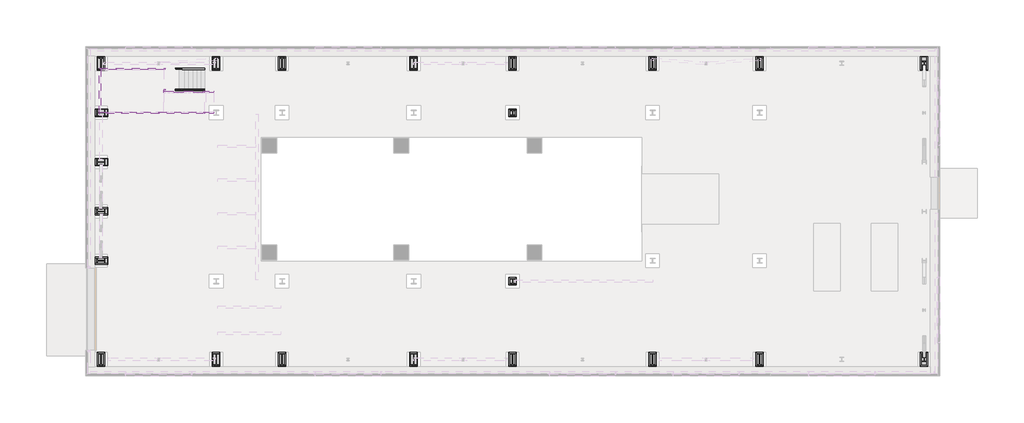
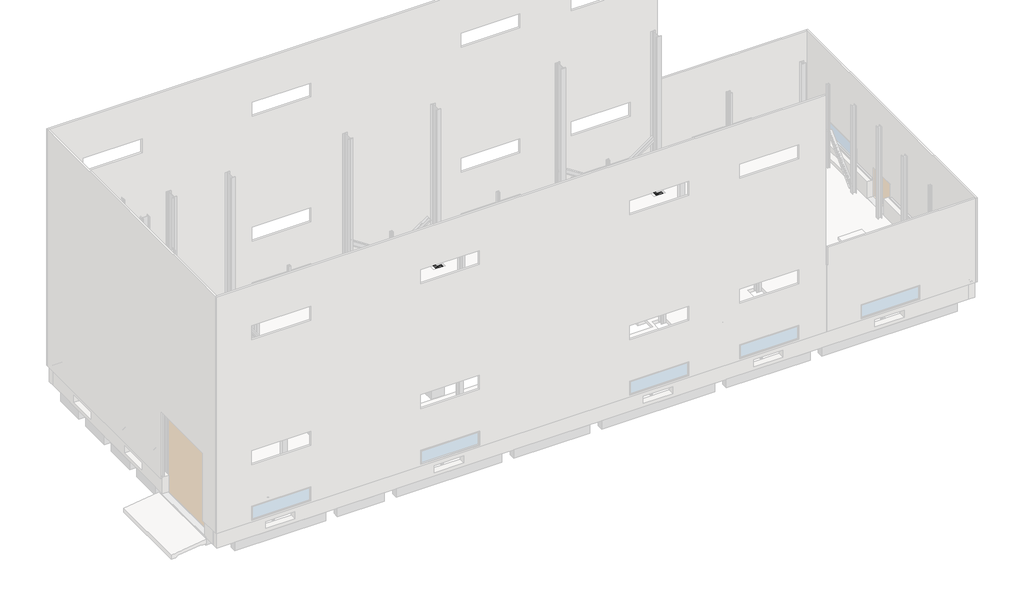
# One storey, part 4 of 4: 23 proxies, 10 members.
"""IFC4 building model written with IfcOpenShell, lengths in millimetres."""

import ifcopenshell
import ifcopenshell.guid

model = None  # the IFC model being written
_history = None  # IfcOwnerHistory: only IFC2X3 demands one
_inside = {}  # id of a spatial element -> (the spatial element, [elements in it])
_under = {}  # id of a project, library or spatial element -> (it, [spatial elements below it])
_declared = {}  # id of a project -> (the project, [libraries it declares])
_typed = {}  # id of a type object -> (the type object, [elements of that type])
_made_of = {}  # id of a material, layer set ... -> (it, [elements and type objects made of it])


def new_model(schema):
    """Start an empty IFC model of exactly this schema.

    Asked for "IFC4X3", IfcOpenShell would pick the latest addendum, in which some entities
    have other attributes; the version numbers below select the first issue.
    IFC2X3 requires an IfcOwnerHistory on every rooted entity: one is made here for all.
    """
    global model, _history
    if schema == "IFC4X3":
        model = ifcopenshell.file(schema_version=(4, 3, 0, 0))
    else:
        model = ifcopenshell.file(schema=schema)
    _inside.clear()
    _under.clear()
    _declared.clear()
    _typed.clear()
    _made_of.clear()
    _history = None
    if model.schema == "IFC2X3":
        org = make("IfcOrganization", Name="unknown")
        user = make(
            "IfcPersonAndOrganization",
            ThePerson=make("IfcPerson", FamilyName="unknown"),
            TheOrganization=org,
        )
        app = make(
            "IfcApplication",
            ApplicationDeveloper=org,
            Version="unknown",
            ApplicationFullName="unknown",
            ApplicationIdentifier="unknown",
        )
        _history = make(
            "IfcOwnerHistory",
            OwningUser=user,
            OwningApplication=app,
            ChangeAction="ADDED",
            CreationDate=0,
        )
    return model


def make(cls, **values):
    """One entity of the class cls with the attributes given. An attribute that is None is left unset."""
    return model.create_entity(
        cls, **{name: value for name, value in values.items() if value is not None}
    )


def rooted(cls, **values):
    """An entity with a GlobalId (a new one), such as an element, a storey or a relation."""
    return make(cls, GlobalId=ifcopenshell.guid.new(), OwnerHistory=_history, **values)


def si_unit(unit_type, name, prefix=None):
    """IfcSIUnit, for example si_unit("LENGTHUNIT", "METRE", prefix="MILLI")."""
    return make("IfcSIUnit", UnitType=unit_type, Prefix=prefix, Name=name)


def assignment(units):
    """IfcUnitAssignment: the units of a project."""
    return None if units is None else make("IfcUnitAssignment", Units=units)


def point(xyz):
    """IfcCartesianPoint."""
    return None if xyz is None else make("IfcCartesianPoint", Coordinates=xyz)


def direction(xyz):
    """IfcDirection."""
    return None if xyz is None else make("IfcDirection", DirectionRatios=xyz)


def frame(location, z_axis=None, x_axis=None):
    """IfcAxis2Placement3D, a coordinate frame: its origin and axes. An axis left out is left unset."""
    return make(
        "IfcAxis2Placement3D",
        Location=point(location),
        Axis=direction(z_axis),
        RefDirection=direction(x_axis),
    )


def frame_2d(location, x_axis=None):
    """IfcAxis2Placement2D, a coordinate frame in the plane: its origin and x axis."""
    return make(
        "IfcAxis2Placement2D", Location=point(location), RefDirection=direction(x_axis)
    )


def origin():
    """The frame at (0, 0, 0) with its axes left unset."""
    return frame((0.0, 0.0, 0.0))


def place(relative_to, where):
    """IfcLocalPlacement: puts the frame where relative to a parent placement (None: the world)."""
    return make(
        "IfcLocalPlacement", PlacementRelTo=relative_to, RelativePlacement=where
    )


def context(
    kind, dimensions, precision=None, world=None, true_north=None, identifier=None
):
    """IfcGeometricRepresentationContext, for example the 3D "Model" context."""
    return make(
        "IfcGeometricRepresentationContext",
        ContextIdentifier=identifier,
        ContextType=kind,
        CoordinateSpaceDimension=dimensions,
        Precision=precision,
        WorldCoordinateSystem=world,
        TrueNorth=true_north,
    )


def project(units=None, contexts=None):
    """IfcProject with its units and contexts."""
    return rooted(
        "IfcProject",
        Name="project",
        RepresentationContexts=contexts,
        UnitsInContext=assignment(units),
    )


def spatial(cls, under=None, at=None, **own):
    """A site, building, storey or space (cls), placed at a placement, below another one or the project."""
    s = rooted(cls, ObjectPlacement=at, **own)
    if under is not None:
        _under.setdefault(under.id(), (under, []))[1].append(s)
    return s


def polyline(points):
    """IfcPolyline through the points."""
    return make("IfcPolyline", Points=[point(p) for p in points])


def circle_curve(where, radius):
    """IfcCircle in the frame where."""
    return make("IfcCircle", Position=where, Radius=radius)


def ellipse_curve(where, semi_axis1, semi_axis2):
    """IfcEllipse in the frame where."""
    return make(
        "IfcEllipse", Position=where, SemiAxis1=semi_axis1, SemiAxis2=semi_axis2
    )


def trimmed(basis, trim1, trim2, sense, master):
    """IfcTrimmedCurve: the piece of a basis curve between two trims."""
    return make(
        "IfcTrimmedCurve",
        BasisCurve=basis,
        Trim1=trim1,
        Trim2=trim2,
        SenseAgreement=sense,
        MasterRepresentation=master,
    )


def segment(curve, same_sense, transition):
    """IfcCompositeCurveSegment."""
    return make(
        "IfcCompositeCurveSegment",
        Transition=transition,
        SameSense=same_sense,
        ParentCurve=curve,
    )


def composite_curve(segments, self_intersect=None):
    """IfcCompositeCurve: segments joined end to end."""
    return make("IfcCompositeCurve", Segments=segments, SelfIntersect=self_intersect)


def outline(outer, holes=None, kind="AREA"):
    """IfcArbitraryClosedProfileDef: a profile drawn as a closed curve; with holes, ...WithVoids."""
    if holes is None:
        return make("IfcArbitraryClosedProfileDef", ProfileType=kind, OuterCurve=outer)
    return make(
        "IfcArbitraryProfileDefWithVoids",
        ProfileType=kind,
        OuterCurve=outer,
        InnerCurves=holes,
    )


def extrude(swept, where, along, depth):
    """IfcExtrudedAreaSolid: the profile swept, set in the frame where, extruded along a direction by depth."""
    return make(
        "IfcExtrudedAreaSolid",
        SweptArea=swept,
        Position=where,
        ExtrudedDirection=direction(along),
        Depth=depth,
    )


def faces_of(points, faces, orient=None, outer=None):
    """IfcFace entities. A face is a list of loops; a loop is a list of indices into points, from 0.

    orient and outer hold one flag for each loop. By default every Orientation is true, the
    first loop of a face is its IfcFaceOuterBound and the others are IfcFaceBound.
    """
    made = []
    for i, loops in enumerate(faces):
        bounds = []
        for j, loop in enumerate(loops):
            is_outer = j == 0 if outer is None else outer[i][j]
            bounds.append(
                make(
                    "IfcFaceOuterBound" if is_outer else "IfcFaceBound",
                    Bound=make("IfcPolyLoop", Polygon=[points[k] for k in loop]),
                    Orientation=True if orient is None else orient[i][j],
                )
            )
        made.append(make("IfcFace", Bounds=bounds))
    return made


def faceted_brep(points, faces, orient=None, outer=None, voids=None):
    """IfcFacetedBrep: a solid bounded by flat faces; with voids (closed shells), ...WithVoids."""
    shared = [point(p) for p in points]
    hull = make("IfcClosedShell", CfsFaces=faces_of(shared, faces, orient, outer))
    if voids is None:
        return make("IfcFacetedBrep", Outer=hull)
    return make(
        "IfcFacetedBrepWithVoids",
        Outer=hull,
        Voids=[
            make(cls, CfsFaces=faces_of(shared, fs, o, b)) for cls, fs, o, b in voids
        ],
    )


def shape(context_of_items, identifier, shape_type, items):
    """IfcShapeRepresentation: the items that make up one representation, for example the "Body"."""
    return make(
        "IfcShapeRepresentation",
        ContextOfItems=context_of_items,
        RepresentationIdentifier=identifier,
        RepresentationType=shape_type,
        Items=items,
    )


def source(mapping_origin, context_of_items, identifier, shape_type, items):
    """IfcRepresentationMap: a shape defined once, which mapped items show again and again."""
    return make(
        "IfcRepresentationMap",
        MappingOrigin=mapping_origin,
        MappedRepresentation=shape(context_of_items, identifier, shape_type, items),
    )


def transform(
    local_origin,
    x_axis=None,
    y_axis=None,
    z_axis=None,
    scale=None,
    scale2=None,
    scale3=None,
    uniform=True,
):
    """IfcCartesianTransformationOperator3D, or its non-uniform kind. x_axis, y_axis, z_axis: its Axis1, 2, 3."""
    if uniform:
        return make(
            "IfcCartesianTransformationOperator3D",
            Axis1=direction(x_axis),
            Axis2=direction(y_axis),
            LocalOrigin=point(local_origin),
            Scale=scale,
            Axis3=direction(z_axis),
        )
    return make(
        "IfcCartesianTransformationOperator3DnonUniform",
        Axis1=direction(x_axis),
        Axis2=direction(y_axis),
        LocalOrigin=point(local_origin),
        Scale=scale,
        Axis3=direction(z_axis),
        Scale2=scale2,
        Scale3=scale3,
    )


def mapped(mapping_source, mapping_target):
    """IfcMappedItem: shows the shape of a source again, moved by a transform."""
    return make(
        "IfcMappedItem", MappingSource=mapping_source, MappingTarget=mapping_target
    )


def made_of(thing, what):
    """Note that an element or type object is made of a material, layer set ...; save() writes the relation."""
    if what is not None:
        _made_of.setdefault(what.id(), (what, []))[1].append(thing)
    return thing


def element(
    cls,
    number,
    at=None,
    inside=None,
    cuts=None,
    type_object=None,
    material=None,
    context=None,
    identifier="Body",
    shape_type=None,
    held_by="IfcProductDefinitionShape",
    body=None,
    shapes=None,
    **own,
):
    """One element of the class cls, such as IfcWall. Its Tag is "e" and its number.

    at: its placement. inside: the storey or other place that contains it. cuts: it is an
    opening in that element (IfcRelVoidsElement). A single representation is given by context,
    identifier, shape_type and body (its items); several are given by shapes. held_by: the class
    of the entity that holds the representations. save() writes the other relations.
    """
    e = rooted(cls, Tag="e%d" % number, ObjectPlacement=at, **own)
    if body is not None:
        shapes = [shape(context, identifier, shape_type, body)]
    if shapes is not None:
        e.Representation = make(held_by, Representations=shapes)
    if inside is not None:
        _inside.setdefault(inside.id(), (inside, []))[1].append(e)
    if cuts is not None:
        rooted(
            "IfcRelVoidsElement", RelatingBuildingElement=cuts, RelatedOpeningElement=e
        )
    if type_object is not None:
        _typed.setdefault(type_object.id(), (type_object, []))[1].append(e)
    return made_of(e, material)


def aggregate(whole, parts):
    """IfcRelAggregates: a whole, such as a stair, and the parts it consists of."""
    return rooted("IfcRelAggregates", RelatingObject=whole, RelatedObjects=parts)


def save(model, path):
    """Write the relations noted so far, then the file.

    IfcRelAggregates (storeys below a building ...), IfcRelContainedInSpatialStructure (elements
    in a storey), IfcRelDefinesByType, IfcRelAssociatesMaterial and IfcRelDeclares: one each for
    every whole, place, type object, material and project.
    """
    for whole, parts in _under.values():
        aggregate(whole, parts)
    for where, things in _inside.values():
        rooted(
            "IfcRelContainedInSpatialStructure",
            RelatedElements=things,
            RelatingStructure=where,
        )
    for kind, things in _typed.values():
        rooted("IfcRelDefinesByType", RelatedObjects=things, RelatingType=kind)
    for what, things in _made_of.values():
        rooted("IfcRelAssociatesMaterial", RelatedObjects=things, RelatingMaterial=what)
    for by, libraries in _declared.values():
        rooted("IfcRelDeclares", RelatingContext=by, RelatedDefinitions=libraries)
    model.write(path)


def plane_surface(at):
    """IfcPlane: the flat surface through the origin of the frame at, square to its z axis."""
    return make("IfcPlane", Position=at)


def cylinder_surface(at, radius):
    """IfcCylindricalSurface: all points at the distance radius from the z axis of the frame at."""
    return make("IfcCylindricalSurface", Position=at, Radius=radius)


def advanced_brep(points, edges, surfaces, faces):
    """IfcAdvancedBrep: a solid bounded by faces that lie on surfaces and meet in shared edges.

    An edge is (start, end): straight between two places in points (the first is 0);
    or (start, end, curve); or (start, end, curve, False) where it runs against its curve.
    A face is (place in surfaces, loops), or (place, loops, False) where it looks against
    its surface's normal. A loop lists edges by number (the first is 1), with a minus sign
    where the edge is run from its end to its start. The first loop is the outer one.
    """
    corners = [point(p) for p in points]
    vertices = [make("IfcVertexPoint", VertexGeometry=c) for c in corners]
    made = []
    for start, end, *more in edges:
        made.append(
            make(
                "IfcEdgeCurve",
                EdgeStart=vertices[start],
                EdgeEnd=vertices[end],
                EdgeGeometry=more[0] if more else make("IfcPolyline", Points=[corners[start], corners[end]]),
                SameSense=more[1] if len(more) > 1 else True,
            )
        )
    hull = []
    for where, loops, *sense in faces:
        bounds = []
        for j, loop in enumerate(loops):
            ring = [make("IfcOrientedEdge", EdgeElement=made[abs(k) - 1], Orientation=k > 0) for k in loop]
            bounds.append(
                make(
                    "IfcFaceOuterBound" if j == 0 else "IfcFaceBound",
                    Bound=make("IfcEdgeLoop", EdgeList=ring),
                    Orientation=True,
                )
            )
        hull.append(make("IfcAdvancedFace", Bounds=bounds, FaceSurface=surfaces[where], SameSense=sense[0] if sense else True))
    return make("IfcAdvancedBrep", Outer=make("IfcClosedShell", CfsFaces=hull))


def generic_models_43c68623(model_context):
    return source(origin(), model_context, "Body", "Brep", [
        faceted_brep([(175.0, 375.0, 863.9720055), (-175.0, 375.0, 863.9720055), (-175.0, -375.0, 863.9720055), (175.0, -375.0, 863.9720055), (225.0, 425.0, 813.9720055), (225.0, -425.0, 813.9720055), (-225.0, -425.0, 813.9720055), (-225.0, 425.0, 813.9720055)], [[[0, 1, 2, 3]], [[4, 5, 6, 7]], [[4, 7, 1, 0]], [[7, 6, 2, 1]], [[6, 5, 3, 2]], [[5, 4, 0, 3]]]),
    ])


def generic_models_49ee4eb4(model_context):
    return source(origin(), model_context, "Body", "Brep", [
        faceted_brep([(25169.0, 25924.5208589, 743.9720055), (24819.0, 25924.5208589, 743.9720055), (24819.0, 25574.5208589, 743.9720055), (25169.0, 25574.5208589, 743.9720055), (25219.0, 25974.5208589, 693.9720055), (25219.0, 25524.5208589, 693.9720055), (24769.0, 25524.5208589, 693.9720055), (24769.0, 25974.5208589, 693.9720055)], [[[0, 1, 2, 3]], [[4, 5, 6, 7]], [[4, 7, 1, 0]], [[7, 6, 2, 1]], [[6, 5, 3, 2]], [[5, 4, 0, 3]]]),
    ])


model = new_model("IFC4")

# Units and contexts
model_context = context("Model", 3, world=origin())
ifc_project = project(units=[si_unit("LENGTHUNIT", "METRE", prefix="MILLI")], contexts=[model_context])

# Site, building, storey
site = spatial("IfcSite", under=ifc_project)
building = spatial("IfcBuilding", under=site)
storey = spatial("IfcBuildingStorey", under=building, Name="1ST T.O.C", Elevation=599.9720055)

# Proxies
placement = place(None, origin())
generic_models_shape = generic_models_43c68623(model_context)
element("IfcBuildingElementProxy", 1, Name="그라우트 : 그라우트", ObjectType="그라우트 : 그라우트", at=placement, inside=storey, context=model_context, shape_type="MappedRepresentation", body=[
    mapped(generic_models_shape, transform((0.0, 20999.5208589, -214.0), x_axis=(1.0, 0.0, 0.0), y_axis=(0.0, 1.0, 0.0), z_axis=(0.0, 0.0, 1.0))),
])
element("IfcBuildingElementProxy", 2, Name="그라우트1 : 그라우트", ObjectType="그라우트1 : 그라우트", at=placement, inside=storey, context=model_context, shape_type="MappedRepresentation", body=[
    mapped(generic_models_shape, transform((6994.0, 20999.5208589, -214.0), x_axis=(1.0, 0.0, 0.0), y_axis=(0.0, 1.0, 0.0), z_axis=(0.0, 0.0, 1.0))),
])
element("IfcBuildingElementProxy", 3, Name="그라우트2 : 그라우트", ObjectType="그라우트2 : 그라우트", at=placement, inside=storey, context=model_context, shape_type="MappedRepresentation", body=[
    mapped(generic_models_shape, transform((6994.0, 20999.5208589, -214.0), x_axis=(1.0, 0.0, 0.0), y_axis=(0.0, 1.0, 0.0), z_axis=(0.0, 0.0, 1.0))),
])
element("IfcBuildingElementProxy", 4, Name="그라우트3 : 그라우트", ObjectType="그라우트3 : 그라우트", at=placement, inside=storey, context=model_context, shape_type="MappedRepresentation", body=[
    mapped(generic_models_shape, transform((10994.0, 20999.5208589, -214.0), x_axis=(1.0, 0.0, 0.0), y_axis=(0.0, 1.0, 0.0), z_axis=(0.0, 0.0, 1.0))),
])
element("IfcBuildingElementProxy", 5, Name="그라우트4 : 그라우트", ObjectType="그라우트4 : 그라우트", at=placement, inside=storey, context=model_context, shape_type="MappedRepresentation", body=[
    mapped(generic_models_shape, transform((18994.0, 20999.5208589, -214.0), x_axis=(1.0, 0.0, 0.0), y_axis=(0.0, 1.0, 0.0), z_axis=(0.0, 0.0, 1.0))),
])
element("IfcBuildingElementProxy", 6, Name="그라우트5 : 그라우트", ObjectType="그라우트5 : 그라우트", at=placement, inside=storey, context=model_context, shape_type="MappedRepresentation", body=[
    mapped(generic_models_shape, transform((24994.0, 20999.5208589, -214.0), x_axis=(1.0, 0.0, 0.0), y_axis=(0.0, 1.0, 0.0), z_axis=(0.0, 0.0, 1.0))),
])
element("IfcBuildingElementProxy", 7, Name="그라우트6 : 그라우트", ObjectType="그라우트6 : 그라우트", at=placement, inside=storey, context=model_context, shape_type="MappedRepresentation", body=[
    mapped(generic_models_shape, transform((33494.0, 20999.5208589, -214.0), x_axis=(1.0, 0.0, 0.0), y_axis=(0.0, 1.0, 0.0), z_axis=(0.0, 0.0, 1.0))),
])
element("IfcBuildingElementProxy", 8, Name="그라우트7 : 그라우트", ObjectType="그라우트7 : 그라우트", at=placement, inside=storey, context=model_context, shape_type="MappedRepresentation", body=[
    mapped(generic_models_shape, transform((39994.0, 20999.5208589, -214.0), x_axis=(1.0, 0.0, 0.0), y_axis=(0.0, 1.0, 0.0), z_axis=(0.0, 0.0, 1.0))),
])
element("IfcBuildingElementProxy", 9, Name="그라우트8 : 그라우트", ObjectType="그라우트8 : 그라우트", at=placement, inside=storey, context=model_context, shape_type="MappedRepresentation", body=[
    mapped(generic_models_shape, transform((39994.0, 38999.5208589, -214.0), x_axis=(1.0, 0.0, 0.0), y_axis=(0.0, 1.0, 0.0), z_axis=(0.0, 0.0, 1.0))),
])
element("IfcBuildingElementProxy", 10, Name="그라우트9 : 그라우트", ObjectType="그라우트9 : 그라우트", at=placement, inside=storey, context=model_context, shape_type="MappedRepresentation", body=[
    mapped(generic_models_shape, transform((33494.0, 38999.5208589, -214.0), x_axis=(1.0, 0.0, 0.0), y_axis=(0.0, 1.0, 0.0), z_axis=(0.0, 0.0, 1.0))),
])
element("IfcBuildingElementProxy", 11, Name="그라우트10 : 그라우트", ObjectType="그라우트10 : 그라우트", at=placement, inside=storey, context=model_context, shape_type="MappedRepresentation", body=[
    mapped(generic_models_shape, transform((24994.0, 38999.5208589, -214.0), x_axis=(1.0, 0.0, 0.0), y_axis=(0.0, 1.0, 0.0), z_axis=(0.0, 0.0, 1.0))),
])
element("IfcBuildingElementProxy", 12, Name="그라우트11 : 그라우트", ObjectType="그라우트11 : 그라우트", at=placement, inside=storey, context=model_context, shape_type="MappedRepresentation", body=[
    mapped(generic_models_shape, transform((18994.0, 38999.5208589, -214.0), x_axis=(1.0, 0.0, 0.0), y_axis=(0.0, 1.0, 0.0), z_axis=(0.0, 0.0, 1.0))),
])
element("IfcBuildingElementProxy", 13, Name="그라우트12 : 그라우트", ObjectType="그라우트12 : 그라우트", at=placement, inside=storey, context=model_context, shape_type="MappedRepresentation", body=[
    mapped(generic_models_shape, transform((10994.0, 38999.5208589, -214.0), x_axis=(1.0, 0.0, 0.0), y_axis=(0.0, 1.0, 0.0), z_axis=(0.0, 0.0, 1.0))),
])
element("IfcBuildingElementProxy", 14, Name="그라우트13 : 그라우트", ObjectType="그라우트13 : 그라우트", at=placement, inside=storey, context=model_context, shape_type="MappedRepresentation", body=[
    mapped(generic_models_shape, transform((6994.0, 38999.5208589, -214.0), x_axis=(1.0, 0.0, 0.0), y_axis=(0.0, 1.0, 0.0), z_axis=(0.0, 0.0, 1.0))),
])
element("IfcBuildingElementProxy", 15, Name="그라우트14 : 그라우트", ObjectType="그라우트14 : 그라우트", at=placement, inside=storey, context=model_context, shape_type="MappedRepresentation", body=[
    mapped(generic_models_shape, transform((-6.0, 38999.5208589, -214.0), x_axis=(1.0, 0.0, 0.0), y_axis=(0.0, 1.0, 0.0), z_axis=(0.0, 0.0, 1.0))),
])
element("IfcBuildingElementProxy", 16, Name="그라우트15 : 그라우트", ObjectType="그라우트15 : 그라우트", at=placement, inside=storey, context=model_context, shape_type="MappedRepresentation", body=[
    mapped(generic_models_shape, transform((-6.0, 35999.5208589, -214.0), x_axis=(0.0, -1.0, 0.0), y_axis=(1.0, 0.0, 0.0), z_axis=(0.0, 0.0, 1.0))),
])
element("IfcBuildingElementProxy", 17, Name="그라우트16 : 그라우트", ObjectType="그라우트16 : 그라우트", at=placement, inside=storey, context=model_context, shape_type="MappedRepresentation", body=[
    mapped(generic_models_shape, transform((-6.0, 32999.5208589, -214.0), x_axis=(0.0, -1.0, 0.0), y_axis=(1.0, 0.0, 0.0), z_axis=(0.0, 0.0, 1.0))),
])
element("IfcBuildingElementProxy", 18, Name="그라우트17 : 그라우트", ObjectType="그라우트17 : 그라우트", at=placement, inside=storey, context=model_context, shape_type="MappedRepresentation", body=[
    mapped(generic_models_shape, transform((-6.0, 29999.5208589, -214.0), x_axis=(0.0, -1.0, 0.0), y_axis=(1.0, 0.0, 0.0), z_axis=(0.0, 0.0, 1.0))),
])
element("IfcBuildingElementProxy", 19, Name="그라우트18 : 그라우트", ObjectType="그라우트18 : 그라우트", at=placement, inside=storey, context=model_context, shape_type="MappedRepresentation", body=[
    mapped(generic_models_shape, transform((-6.0, 26999.5208589, -214.0), x_axis=(0.0, -1.0, 0.0), y_axis=(1.0, 0.0, 0.0), z_axis=(0.0, 0.0, 1.0))),
])
element("IfcBuildingElementProxy", 20, Name="그라우트20 : 그라우트", ObjectType="그라우트20 : 그라우트", at=placement, inside=storey, context=model_context, shape_type="MappedRepresentation", body=[
    mapped(generic_models_shape, transform((49994.0, 38999.5208589, -214.0), x_axis=(1.0, 0.0, 0.0), y_axis=(0.0, 1.0, 0.0), z_axis=(0.0, 0.0, 1.0))),
])
element("IfcBuildingElementProxy", 21, Name="그라우트22 : 그라우트", ObjectType="그라우트22 : 그라우트", at=placement, inside=storey, context=model_context, shape_type="MappedRepresentation", body=[
    mapped(generic_models_shape, transform((49994.0, 20999.5208589, -214.0), x_axis=(1.0, 0.0, 0.0), y_axis=(0.0, 1.0, 0.0), z_axis=(0.0, 0.0, 1.0))),
])
generic_models_2_shape = generic_models_49ee4eb4(model_context)
element("IfcBuildingElementProxy", 22, Name="그라우트23 : 그라우트", ObjectType="그라우트23 : 그라우트", at=placement, inside=storey, context=model_context, shape_type="MappedRepresentation", body=[
    mapped(generic_models_2_shape, transform((0.0, 0.0, -94.0), x_axis=(1.0, 0.0, 0.0), y_axis=(0.0, 1.0, 0.0), z_axis=(0.0, 0.0, 1.0))),
])
element("IfcBuildingElementProxy", 23, Name="그라우트19 : 그라우트", ObjectType="그라우트19 : 그라우트", at=placement, inside=storey, context=model_context, shape_type="MappedRepresentation", body=[
    mapped(generic_models_2_shape, transform((0.0, 10250.0, -94.0), x_axis=(1.0, 0.0, 0.0), y_axis=(0.0, 1.0, 0.0), z_axis=(0.0, 0.0, 1.0))),
])

# Members
element("IfcMember", 24, ObjectType="C-250X90", at=placement, inside=storey, context=model_context, shape_type="AdvancedBrep", body=[
    advanced_brep(
    [(6309.5374538, 37424.5208589, 599.9720055), (6309.5374538, 37413.5208589, 599.9720055), (6192.9345962, 37413.5208589, 599.9720055), (6174.6503035, 37345.6208589, 599.9720055), (6155.7782632, 37334.5208589, 599.9720055), (6155.7782632, 37424.5208589, 599.9720055), (6309.5374538, 37424.5208589, 797.2714693), (6309.5374538, 37334.5208589, 797.2714693), (6309.5374538, 37345.6208589, 783.5463491), (6309.5374538, 37413.5208589, 770.2486816), (3899.5374538, 37424.5208589, 2240.8744123), (3899.5374538, 37424.5208589, 2549.998742), (3899.5374538, 37345.6208589, 2536.2736218), (3899.5374538, 37413.5208589, 2522.9759544), (3899.5374538, 37334.5208589, 2549.998742), (3899.5374538, 37334.5208589, 2240.8744123), (3899.5374538, 37345.6208589, 2254.5995325), (3899.5374538, 37413.5208589, 2267.8972)],
    [
        (0, 1),
        (1, 2),
        (2, 3),
        (3, 4, ellipse_curve(frame((6155.7782632, 37345.6208589, 599.9720055), z_axis=(0.0, 0.0, -1.0), x_axis=(1.0, 0.0, 0.0)), 18.8720403, 11.1)),
        (4, 5),
        (5, 0),
        (6, 7),
        (7, 8, ellipse_curve(frame((6309.5374538, 37345.6208589, 797.2714693), z_axis=(1.0, 0.0, 0.0), x_axis=(0.0, 0.0, -0.9999999999999999)), 13.7251202, 11.1)),
        (8, 9),
        (9, 1),
        (0, 6),
        (5, 10),
        (10, 11),
        (11, 6),
        (8, 12),
        (12, 13),
        (13, 9),
        (7, 14),
        (14, 12, ellipse_curve(frame((3899.5374538, 37345.6208589, 2549.998742), z_axis=(1.0, 0.0, 0.0), x_axis=(0.0, 0.0, -0.9999999999999999)), 13.7251202, 11.1)),
        (11, 14),
        (4, 15),
        (15, 10),
        (3, 16),
        (16, 15, ellipse_curve(frame((3899.5374538, 37345.6208589, 2240.8744123), z_axis=(1.0, 0.0, 0.0), x_axis=(0.0, 0.0, -0.9999999999999999)), 13.7251202, 11.1)),
        (2, 17),
        (17, 16),
        (13, 17),
    ],
    [
        plane_surface(frame((0.0, 0.0, 599.9720055), z_axis=(0.0, 0.0, -1.0), x_axis=(1.0, 0.0, 0.0))),
        plane_surface(frame((6309.5374538, 37424.5208589, 797.2714693), z_axis=(1.0, 0.0, 0.0), x_axis=(0.0, -1.0, 0.0))),
        plane_surface(frame((6309.5374538, 37424.5208589, 488.1471396), z_axis=(0.0, 1.0, 0.0), x_axis=(-0.8087360843031884, 0.0, 0.5881716976750463))),
        plane_surface(frame((6309.5374538, 37345.6208589, 783.5463491), z_axis=(-0.5809303280616924, -0.15643446504022573, -0.7987792010848263), x_axis=(-0.8087360843031886, 0.0, 0.5881716976750463))),
        cylinder_surface(frame((6309.5374538, 37345.6208589, 797.2714693), z_axis=(0.8087360843031884, 0.0, -0.5881716976750463), x_axis=(0.0, -1.0, 0.0)), 11.1),
        plane_surface(frame((6309.5374538, 37424.5208589, 797.2714693), z_axis=(0.5881716976750463, 0.0, 0.8087360843031886), x_axis=(-0.8087360843031886, 0.0, 0.5881716976750463))),
        plane_surface(frame((6309.5374538, 37334.5208589, 488.1471396), z_axis=(-0.5881716976750463, 0.0, -0.8087360843031884), x_axis=(-0.8087360843031884, 0.0, 0.5881716976750463))),
        cylinder_surface(frame((6162.4945294, 37345.6208589, 595.0874482), z_axis=(0.8087360843031884, 0.0, -0.5881716976750463), x_axis=(0.0, -1.0, 0.0)), 11.1),
        plane_surface(frame((6309.5374538, 37413.5208589, 515.1699273), z_axis=(0.5809303280616908, -0.15643446504023575, 0.7987792010848253), x_axis=(-0.8087360843031884, 0.0, 0.5881716976750463))),
        plane_surface(frame((6309.5374538, 37413.5208589, 770.2486816), z_axis=(0.0, -1.0, 0.0), x_axis=(-0.8087360843031884, 0.0, 0.5881716976750463))),
        plane_surface(frame((3899.5374538, 37328.5647627, 2426.9720055), z_axis=(-1.0, 0.0, 0.0), x_axis=(0.0, 1.0, 0.0))),
    ],
    [
        (0, [[1, 2, 3, 4, 5, 6]]),
        (1, [[7, 8, 9, 10, -1, 11]]),
        (2, [[-11, -6, 12, 13, 14]]),
        (3, [[-9, 15, 16, 17]]),
        (4, [[-8, 18, 19, -15]]),
        (5, [[-7, -14, 20, -18]]),
        (6, [[21, 22, -12, -5]]),
        (7, [[23, 24, -21, -4]]),
        (8, [[25, 26, -23, -3]]),
        (9, [[-10, -17, 27, -25, -2]]),
        (10, [[-13, -22, -24, -26, -27, -16, -19, -20]]),
    ],
),
])
element("IfcMember", 25, ObjectType="C-250X90", at=placement, inside=storey, context=model_context, shape_type="AdvancedBrep", body=[
    advanced_brep(
    [(6309.5374538, 38635.5208589, 599.9720055), (6309.5374538, 38624.5208589, 599.9720055), (6155.7782632, 38624.5208589, 599.9720055), (6155.7782632, 38714.5208589, 599.9720055), (6174.6503035, 38703.4208589, 599.9720055), (6192.9345962, 38635.5208589, 599.9720055), (6309.5374538, 38624.5208589, 797.2714693), (6309.5374538, 38635.5208589, 770.2486816), (6309.5374538, 38703.4208589, 783.5463491), (6309.5374538, 38714.5208589, 797.2714693), (3899.5742166, 38624.5208589, 2549.9720055), (3818.2782632, 38624.5208589, 2299.9720055), (3899.5742166, 38714.5208589, 2549.9720055), (3895.9646762, 38703.4208589, 2538.8720055), (3892.4675508, 38635.5208589, 2528.117702), (3818.2782632, 38714.5208589, 2299.9720055), (3821.8878035, 38703.4208589, 2311.0720055), (3825.3849289, 38635.5208589, 2321.826309)],
    [
        (0, 1),
        (1, 2),
        (2, 3),
        (3, 4, ellipse_curve(frame((6155.7782632, 38703.4208589, 599.9720055), z_axis=(0.0, 0.0, -1.0), x_axis=(1.0, 0.0, 0.0)), 18.8720403, 11.1)),
        (4, 5),
        (5, 0),
        (6, 1),
        (0, 7),
        (7, 8),
        (8, 9, ellipse_curve(frame((6309.5374538, 38703.4208589, 797.2714693), z_axis=(1.0, 0.0, 0.0), x_axis=(0.0, 0.0, -0.9999999999999999)), 13.7251202, 11.1)),
        (9, 6),
        (6, 10),
        (10, 11),
        (11, 2),
        (9, 12),
        (12, 10),
        (8, 13),
        (13, 12, ellipse_curve(frame((3899.5742166, 38703.4208589, 2549.9720055), z_axis=(0.9509826718461247, 0.0, -0.30924417189076664), x_axis=(-0.30924417189076714, 0.0, -0.9509826718461244)), 11.672137, 11.1)),
        (7, 14),
        (14, 13),
        (11, 15),
        (15, 3),
        (4, 16),
        (16, 17),
        (17, 5),
        (15, 16, ellipse_curve(frame((3818.2782632, 38703.4208589, 2299.9720055), z_axis=(0.9509826718461247, 0.0, -0.30924417189076664), x_axis=(-0.30924417189076714, 0.0, -0.9509826718461244)), 11.672137, 11.1)),
        (17, 14),
    ],
    [
        plane_surface(frame((0.0, 0.0, 599.9720055), z_axis=(0.0, 0.0, -1.0), x_axis=(1.0, 0.0, 0.0))),
        plane_surface(frame((6309.5374538, 38624.5208589, 797.2714693), z_axis=(1.0, 0.0, 0.0), x_axis=(0.0, -1.0, 0.0))),
        plane_surface(frame((6309.5374538, 38624.5208589, 797.2714693), z_axis=(0.0, -1.0000000000000002, 0.0), x_axis=(-0.8087360843031886, 0.0, 0.5881716976750463))),
        plane_surface(frame((6309.5374538, 38714.5208589, 797.2714693), z_axis=(0.5881716976750463, 0.0, 0.8087360843031886), x_axis=(-0.8087360843031886, 0.0, 0.5881716976750463))),
        cylinder_surface(frame((6309.5374538, 38703.4208589, 797.2714693), z_axis=(0.8087360843031884, 0.0, -0.5881716976750463), x_axis=(0.0, 1.0, 0.0)), 11.1),
        plane_surface(frame((6309.5374538, 38635.5208589, 770.2486816), z_axis=(-0.5809303280616913, 0.15643446504022976, -0.798779201084826), x_axis=(-0.8087360843031884, 0.0, 0.5881716976750463))),
        plane_surface(frame((6309.5374538, 38624.5208589, 488.1471396), z_axis=(-0.5881716976750463, 0.0, -0.8087360843031884), x_axis=(-0.8087360843031884, 0.0, 0.5881716976750463))),
        plane_surface(frame((6309.5374538, 38703.4208589, 501.8722598), z_axis=(0.5809303280616918, 0.1564344650402317, 0.7987792010848254), x_axis=(-0.8087360843031884, 0.0, 0.5881716976750463))),
        cylinder_surface(frame((6162.4945294, 38703.4208589, 595.0874482), z_axis=(0.8087360843031884, 0.0, -0.5881716976750463), x_axis=(0.0, 1.0, 0.0)), 11.1),
        plane_surface(frame((6309.5374538, 38635.5208589, 515.1699273), z_axis=(0.0, 1.0000000000000002, 0.0), x_axis=(-0.8087360843031886, 0.0, 0.5881716976750463))),
        plane_surface(frame((3899.5742166, 38624.5208589, 2549.9720055), z_axis=(-0.9509826718461247, 0.0, 0.30924417189076664), x_axis=(0.0, 1.0, 0.0))),
    ],
    [
        (0, [[1, 2, 3, 4, 5, 6]]),
        (1, [[7, -1, 8, 9, 10, 11]]),
        (2, [[-7, 12, 13, 14, -2]]),
        (3, [[-11, 15, 16, -12]]),
        (4, [[-10, 17, 18, -15]]),
        (5, [[-9, 19, 20, -17]]),
        (6, [[-14, 21, 22, -3]]),
        (7, [[23, 24, 25, -5]]),
        (8, [[-22, 26, -23, -4]]),
        (9, [[-8, -6, -25, 27, -19]]),
        (10, [[-16, -18, -20, -27, -24, -26, -21, -13]]),
    ],
),
])
element("IfcMember", 26, ObjectType="C-250X90", at=placement, inside=storey, context=model_context, shape_type="AdvancedBrep", body=[
    advanced_brep(
    [(3809.5374538, 37232.6086665, 2797.2714693), (3809.5374538, 37232.6086665, 2488.1471396), (6300.7966445, 37232.6086665, 4299.9720055), (6219.5006911, 37232.6086665, 4549.9720055), (3809.5374538, 37322.6086665, 2488.1471396), (6300.7966445, 37322.6086665, 4299.9720055), (3809.5374538, 37311.5086665, 2501.8722598), (6297.1871042, 37311.5086665, 4311.0720055), (3809.5374538, 37243.6086665, 2515.1699273), (6293.6899788, 37243.6086665, 4321.826309), (3809.5374538, 37243.6086665, 2770.2486816), (3809.5374538, 37311.5086665, 2783.5463491), (6223.1102315, 37311.5086665, 4538.8720055), (6226.6073569, 37243.6086665, 4528.117702), (3809.5374538, 37322.6086665, 2797.2714693), (6219.5006911, 37322.6086665, 4549.9720055)],
    [
        (0, 1),
        (1, 2),
        (2, 3),
        (3, 0),
        (1, 4),
        (4, 5),
        (5, 2),
        (4, 6, ellipse_curve(frame((3809.5374538, 37311.5086665, 2488.1471396), z_axis=(1.0, 0.0, 0.0), x_axis=(0.0, 0.0, -1.0)), 13.7251202, 11.1)),
        (6, 7),
        (7, 5, ellipse_curve(frame((6300.7966445, 37311.5086665, 4299.9720055), z_axis=(-0.9509826718461247, 0.0, -0.30924417189076625), x_axis=(0.3092441718907662, 0.0, -0.9509826718461247)), 11.672137, 11.1)),
        (6, 8),
        (8, 9),
        (9, 7),
        (10, 11),
        (11, 12),
        (12, 13),
        (13, 10),
        (11, 14, ellipse_curve(frame((3809.5374538, 37311.5086665, 2797.2714693), z_axis=(1.0, 0.0, 0.0), x_axis=(0.0, 0.0, -1.0)), 13.7251202, 11.1)),
        (14, 15),
        (15, 12, ellipse_curve(frame((6219.5006911, 37311.5086665, 4549.9720055), z_axis=(-0.9509826718461247, 0.0, -0.30924417189076625), x_axis=(0.3092441718907662, 0.0, -0.9509826718461247)), 11.672137, 11.1)),
        (14, 0),
        (3, 15),
        (8, 10),
        (13, 9),
    ],
    [
        plane_surface(frame((3809.5374538, 37232.6086665, 2488.1471396), z_axis=(0.0, -1.0, 0.0), x_axis=(0.8087360843031883, 0.0, 0.5881716976750465))),
        plane_surface(frame((3809.5374538, 37322.6086665, 2488.1471396), z_axis=(0.5881716976750465, 0.0, -0.8087360843031883), x_axis=(0.8087360843031883, 0.0, 0.5881716976750465))),
        cylinder_surface(frame((3956.5803783, 37311.5086665, 2595.0874482), z_axis=(-0.8087360843031883, 0.0, -0.5881716976750465), x_axis=(0.0, 1.0, 0.0)), 11.1),
        plane_surface(frame((3809.5374538, 37243.6086665, 2515.1699273), z_axis=(-0.5809303280616911, 0.15643446504023578, 0.798779201084825), x_axis=(0.8087360843031882, 0.0, 0.5881716976750466))),
        plane_surface(frame((3809.5374538, 37311.5086665, 2783.5463491), z_axis=(0.5809303280616926, 0.15643446504022573, -0.798779201084826), x_axis=(0.8087360843031883, 0.0, 0.5881716976750465))),
        cylinder_surface(frame((3809.5374538, 37311.5086665, 2797.2714693), z_axis=(-0.8087360843031883, 0.0, -0.5881716976750465), x_axis=(0.0, 1.0, 0.0)), 11.1),
        plane_surface(frame((3809.5374538, 37232.6086665, 2797.2714693), z_axis=(-0.5881716976750465, 0.0, 0.8087360843031883), x_axis=(0.8087360843031883, 0.0, 0.5881716976750465))),
        plane_surface(frame((3809.5374538, 37243.6086665, 2770.2486816), z_axis=(0.0, 1.0, 0.0), x_axis=(0.8087360843031883, 0.0, 0.5881716976750465))),
        plane_surface(frame((3809.5374538, 37328.5647627, 2426.9720055), z_axis=(-1.0, 0.0, 0.0), x_axis=(0.0, 1.0, 0.0))),
        plane_surface(frame((6219.5006911, 37282.6086665, 4549.9720055), z_axis=(0.9509826718461247, 0.0, 0.30924417189076625), x_axis=(0.0, -1.0, 0.0))),
    ],
    [
        (0, [[1, 2, 3, 4]]),
        (1, [[5, 6, 7, -2]]),
        (2, [[8, 9, 10, -6]]),
        (3, [[11, 12, 13, -9]]),
        (4, [[14, 15, 16, 17]]),
        (5, [[18, 19, 20, -15]]),
        (6, [[21, -4, 22, -19]]),
        (7, [[23, -17, 24, -12]]),
        (8, [[-21, -18, -14, -23, -11, -8, -5, -1]]),
        (9, [[-3, -7, -10, -13, -24, -16, -20, -22]]),
    ],
),
])
element("IfcMember", 27, ObjectType="C-250X90", at=placement, inside=storey, context=model_context, shape_type="AdvancedBrep", body=[
    advanced_brep(
    [(3550.7966445, 36032.6086665, 2299.9720055), (3469.5006911, 36032.6086665, 2549.9720055), (6219.5006911, 36032.6086665, 4549.9720055), (6300.7966445, 36032.6086665, 4299.9720055), (3469.5006911, 35942.6086665, 2549.9720055), (6219.5006911, 35942.6086665, 4549.9720055), (3473.1102315, 35953.7086665, 2538.8720055), (6223.1102315, 35953.7086665, 4538.8720055), (3476.6073569, 36021.6086665, 2528.117702), (6226.6073569, 36021.6086665, 4528.117702), (3543.6899788, 36021.6086665, 2321.826309), (3547.1871042, 35953.7086665, 2311.0720055), (6297.1871042, 35953.7086665, 4311.0720055), (6293.6899788, 36021.6086665, 4321.826309), (3550.7966445, 35942.6086665, 2299.9720055), (6300.7966445, 35942.6086665, 4299.9720055)],
    [
        (0, 1),
        (1, 2),
        (2, 3),
        (3, 0),
        (1, 4),
        (4, 5),
        (5, 2),
        (4, 6, ellipse_curve(frame((3469.5006911, 35953.7086665, 2549.9720055), z_axis=(0.9509826718461252, 0.0, 0.30924417189076514), x_axis=(0.3092441718907655, 0.0, -0.9509826718461252)), 11.672137, 11.1)),
        (6, 7),
        (7, 5, ellipse_curve(frame((6219.5006911, 35953.7086665, 4549.9720055), z_axis=(-0.9509826718461247, 0.0, -0.30924417189076625), x_axis=(0.3092441718907662, 0.0, -0.9509826718461247)), 11.672137, 11.1)),
        (6, 8),
        (8, 9),
        (9, 7),
        (10, 11),
        (11, 12),
        (12, 13),
        (13, 10),
        (11, 14, ellipse_curve(frame((3550.7966445, 35953.7086665, 2299.9720055), z_axis=(0.9509826718461252, 0.0, 0.30924417189076514), x_axis=(0.3092441718907655, 0.0, -0.9509826718461252)), 11.672137, 11.1)),
        (14, 15),
        (15, 12, ellipse_curve(frame((6300.7966445, 35953.7086665, 4299.9720055), z_axis=(-0.9509826718461247, 0.0, -0.30924417189076625), x_axis=(0.3092441718907662, 0.0, -0.9509826718461247)), 11.672137, 11.1)),
        (14, 0),
        (3, 15),
        (8, 10),
        (13, 9),
    ],
    [
        plane_surface(frame((3809.5374538, 36032.6086665, 2797.2714693), z_axis=(0.0, 1.0, 0.0), x_axis=(0.8087360843031883, 0.0, 0.5881716976750465))),
        plane_surface(frame((3809.5374538, 35942.6086665, 2797.2714693), z_axis=(-0.5881716976750465, 0.0, 0.8087360843031883), x_axis=(0.8087360843031883, 0.0, 0.5881716976750465))),
        cylinder_surface(frame((3809.5374538, 35953.7086665, 2797.2714693), z_axis=(-0.8087360843031883, 0.0, -0.5881716976750465), x_axis=(0.0, -1.0, 0.0)), 11.1),
        plane_surface(frame((3809.5374538, 36021.6086665, 2770.2486816), z_axis=(0.5809303280616915, -0.1564344650402298, -0.7987792010848259), x_axis=(0.8087360843031883, 0.0, 0.5881716976750465))),
        plane_surface(frame((3809.5374538, 35953.7086665, 2501.8722598), z_axis=(-0.5809303280616922, -0.15643446504023178, 0.7987792010848251), x_axis=(0.8087360843031882, 0.0, 0.5881716976750466))),
        cylinder_surface(frame((3956.5803783, 35953.7086665, 2595.0874482), z_axis=(-0.8087360843031883, 0.0, -0.5881716976750465), x_axis=(0.0, -1.0, 0.0)), 11.1),
        plane_surface(frame((3809.5374538, 36032.6086665, 2488.1471396), z_axis=(0.5881716976750465, 0.0, -0.8087360843031883), x_axis=(0.8087360843031883, 0.0, 0.5881716976750465))),
        plane_surface(frame((3809.5374538, 36021.6086665, 2515.1699273), z_axis=(0.0, -1.0, 0.0), x_axis=(0.8087360843031882, 0.0, 0.5881716976750466))),
        plane_surface(frame((3469.5006911, 36032.6086665, 2549.9720055), z_axis=(-0.9509826718461252, 0.0, -0.30924417189076514), x_axis=(0.0, -1.0, 0.0))),
        plane_surface(frame((6219.5006911, 36032.6086665, 4549.9720055), z_axis=(0.9509826718461247, 0.0, 0.30924417189076625), x_axis=(0.0, -1.0, 0.0))),
    ],
    [
        (0, [[1, 2, 3, 4]]),
        (1, [[5, 6, 7, -2]]),
        (2, [[8, 9, 10, -6]]),
        (3, [[11, 12, 13, -9]]),
        (4, [[14, 15, 16, 17]]),
        (5, [[18, 19, 20, -15]]),
        (6, [[21, -4, 22, -19]]),
        (7, [[23, -17, 24, -12]]),
        (8, [[-1, -21, -18, -14, -23, -11, -8, -5]]),
        (9, [[-7, -10, -13, -24, -16, -20, -22, -3]]),
    ],
),
])
element("IfcMember", 28, ObjectType="C-250X90", at=placement, inside=storey, context=model_context, shape_type="SweptSolid", body=[
    extrude(outline(composite_curve([segment(polyline([(2549.9720055, 3809.5374538), (2299.9720055, 3809.5374538), (2299.9720055, 3899.5374538)]), True, "CONTINUOUS"), segment(trimmed(circle_curve(frame_2d((2299.9720055, 3888.4374538)), 11.1), [point((2299.9720055, 3899.5374538))], [point((2311.0720055, 3888.4374538))], False, "CARTESIAN"), True, "CONTINUOUS"), segment(polyline([(2311.0720055, 3888.4374538), (2321.826309, 3820.5374538), (2528.117702, 3820.5374538), (2538.8720055, 3888.4374538)]), True, "CONTINUOUS"), segment(trimmed(circle_curve(frame_2d((2549.9720055, 3888.4374538)), 11.1), [point((2538.8720055, 3888.4374538))], [point((2549.9720055, 3899.5374538))], False, "CARTESIAN"), True, "CONTINUOUS"), segment(polyline([(2549.9720055, 3899.5374538), (2549.9720055, 3809.5374538)]), True, "CONTINUOUS")], self_intersect=False)), frame((0.0, 37322.6086665, 0.0), z_axis=(0.0, 1.0, 0.0), x_axis=(0.0, 0.0, 1.0)), (0.0, 0.0, 1.0), 101.9121924),
])
element("IfcMember", 29, ObjectType="C-250X90", at=placement, inside=storey, context=model_context, shape_type="AdvancedBrep", body=[
    advanced_brep(
    [(3818.2782632, 38624.5208589, 2299.9720055), (3899.5742166, 38624.5208589, 2549.9720055), (0.0, 38624.5208589, 2549.9720055), (0.0, 38624.5208589, 2299.9720055), (3899.5742166, 38714.5208589, 2549.9720055), (-90.0, 38714.5208589, 2549.9720055), (3895.9646762, 38703.4208589, 2538.8720055), (-78.9, 38703.4208589, 2538.8720055), (3892.4675508, 38635.5208589, 2528.117702), (-11.0, 38635.5208589, 2528.117702), (3825.3849289, 38635.5208589, 2321.826309), (3821.8878035, 38703.4208589, 2311.0720055), (-78.9, 38703.4208589, 2311.0720055), (-11.0, 38635.5208589, 2321.826309), (3818.2782632, 38714.5208589, 2299.9720055), (-90.0, 38714.5208589, 2299.9720055)],
    [
        (0, 1),
        (1, 2),
        (2, 3),
        (3, 0),
        (1, 4),
        (4, 5),
        (5, 2),
        (4, 6, ellipse_curve(frame((3899.5742166, 38703.4208589, 2549.9720055), z_axis=(-0.9509826718461252, 0.0, 0.30924417189076514), x_axis=(0.30924417189076503, 0.0, 0.9509826718461252)), 11.672137, 11.1)),
        (6, 7),
        (7, 5, ellipse_curve(frame((-78.9, 38703.4208589, 2549.9720055), z_axis=(0.7071067811865591, 0.707106781186536, 0.0), x_axis=(0.7071067811865358, -0.7071067811865591, 0.0)), 15.6977705, 11.1)),
        (6, 8),
        (8, 9),
        (9, 7),
        (10, 11),
        (11, 12),
        (12, 13),
        (13, 10),
        (11, 14, ellipse_curve(frame((3818.2782632, 38703.4208589, 2299.9720055), z_axis=(-0.9509826718461252, 0.0, 0.30924417189076514), x_axis=(0.30924417189076503, 0.0, 0.9509826718461252)), 11.672137, 11.1)),
        (14, 15),
        (15, 12, ellipse_curve(frame((-78.9, 38703.4208589, 2299.9720055), z_axis=(0.7071067811865591, 0.707106781186536, 0.0), x_axis=(0.7071067811865358, -0.7071067811865591, 0.0)), 15.6977705, 11.1)),
        (14, 0),
        (3, 15),
        (8, 10),
        (13, 9),
    ],
    [
        plane_surface(frame((3809.5374538, 38624.5208589, 2549.9720055), z_axis=(0.0, -1.0, 0.0), x_axis=(-1.0, 0.0, 0.0))),
        plane_surface(frame((3809.5374538, 38714.5208589, 2549.9720055), z_axis=(0.0, 0.0, 1.0), x_axis=(-1.0, 0.0, 0.0))),
        cylinder_surface(frame((3809.5374538, 38703.4208589, 2549.9720055), z_axis=(1.0, 0.0, 0.0), x_axis=(0.0, 1.0, 0.0)), 11.1),
        plane_surface(frame((3809.5374538, 38635.5208589, 2528.117702), z_axis=(0.0, 0.15643446504022773, -0.9876883405951383), x_axis=(-1.0, 0.0, 0.0))),
        plane_surface(frame((3809.5374538, 38703.4208589, 2311.0720055), z_axis=(0.0, 0.15643446504023373, 0.9876883405951373), x_axis=(-1.0, 0.0, 0.0))),
        cylinder_surface(frame((3809.5374538, 38703.4208589, 2299.9720055), z_axis=(1.0, 0.0, 0.0), x_axis=(0.0, 1.0, 0.0)), 11.1),
        plane_surface(frame((3809.5374538, 38624.5208589, 2299.9720055), z_axis=(0.0, 0.0, -1.0), x_axis=(-1.0, 0.0, 0.0))),
        plane_surface(frame((3809.5374538, 38635.5208589, 2321.826309), z_axis=(0.0, 1.0, 0.0), x_axis=(-1.0, 0.0, 0.0))),
        plane_surface(frame((3899.5742166, 38624.5208589, 2549.9720055), z_axis=(0.9509826718461252, 0.0, -0.30924417189076514), x_axis=(0.0, 1.0, 0.0))),
        plane_surface(frame((0.0, 38624.5208589, 2549.9720055), z_axis=(-0.7071067811865591, -0.707106781186536, 0.0), x_axis=(-0.707106781186536, 0.7071067811865591, 0.0))),
    ],
    [
        (0, [[1, 2, 3, 4]]),
        (1, [[5, 6, 7, -2]]),
        (2, [[8, 9, 10, -6]]),
        (3, [[11, 12, 13, -9]]),
        (4, [[14, 15, 16, 17]]),
        (5, [[18, 19, 20, -15]]),
        (6, [[21, -4, 22, -19]]),
        (7, [[23, -17, 24, -12]]),
        (8, [[-1, -21, -18, -14, -23, -11, -8, -5]]),
        (9, [[-7, -10, -13, -24, -16, -20, -22, -3]]),
    ],
),
])
element("IfcMember", 30, ObjectType="C-250X90", at=placement, inside=storey, context=model_context, shape_type="AdvancedBrep", body=[
    advanced_brep(
    [(0.0, 38624.5208589, 2299.9720055), (0.0, 38624.5208589, 2549.9720055), (0.0, 36032.6086665, 2549.9720055), (0.0, 36032.6086665, 2299.9720055), (-90.0, 38714.5208589, 2549.9720055), (-90.0, 35942.6086665, 2549.9720055), (-78.9, 38703.4208589, 2538.8720055), (-78.9, 35953.7086665, 2538.8720055), (-11.0, 38635.5208589, 2528.117702), (-11.0, 36021.6086665, 2528.117702), (-11.0, 38635.5208589, 2321.826309), (-78.9, 38703.4208589, 2311.0720055), (-78.9, 35953.7086665, 2311.0720055), (-11.0, 36021.6086665, 2321.826309), (-90.0, 38714.5208589, 2299.9720055), (-90.0, 35942.6086665, 2299.9720055)],
    [
        (0, 1),
        (1, 2),
        (2, 3),
        (3, 0),
        (1, 4),
        (4, 5),
        (5, 2),
        (4, 6, ellipse_curve(frame((-78.9, 38703.4208589, 2549.9720055), z_axis=(-0.7071067811865591, -0.707106781186536, 0.0), x_axis=(-0.707106781186536, 0.7071067811865588, 0.0)), 15.6977705, 11.1)),
        (6, 7),
        (7, 5, ellipse_curve(frame((-78.9, 35953.7086665, 2549.9720055), z_axis=(-0.7071067811865591, 0.707106781186536, 0.0), x_axis=(0.707106781186536, 0.7071067811865588, 0.0)), 15.6977705, 11.1)),
        (6, 8),
        (8, 9),
        (9, 7),
        (10, 11),
        (11, 12),
        (12, 13),
        (13, 10),
        (11, 14, ellipse_curve(frame((-78.9, 38703.4208589, 2299.9720055), z_axis=(-0.7071067811865591, -0.707106781186536, 0.0), x_axis=(-0.707106781186536, 0.7071067811865588, 0.0)), 15.6977705, 11.1)),
        (14, 15),
        (15, 12, ellipse_curve(frame((-78.9, 35953.7086665, 2299.9720055), z_axis=(-0.7071067811865591, 0.707106781186536, 0.0), x_axis=(0.707106781186536, 0.7071067811865588, 0.0)), 15.6977705, 11.1)),
        (14, 0),
        (3, 15),
        (8, 10),
        (13, 9),
    ],
    [
        plane_surface(frame((0.0, 38624.5208589, 2549.9720055), z_axis=(1.0, 0.0, 0.0), x_axis=(0.0, -1.0, 0.0))),
        plane_surface(frame((-90.0, 38624.5208589, 2549.9720055), z_axis=(0.0, 0.0, 1.0), x_axis=(0.0, -1.0, 0.0))),
        cylinder_surface(frame((-78.9, 38624.5208589, 2549.9720055), z_axis=(0.0, 1.0, 0.0), x_axis=(-1.0, 0.0, 0.0)), 11.1),
        plane_surface(frame((-11.0, 38624.5208589, 2528.117702), z_axis=(-0.15643446504022773, 0.0, -0.9876883405951383), x_axis=(0.0, -1.0, 0.0))),
        plane_surface(frame((-78.9, 38624.5208589, 2311.0720055), z_axis=(-0.15643446504023373, 0.0, 0.9876883405951373), x_axis=(0.0, -1.0, 0.0))),
        cylinder_surface(frame((-78.9, 38624.5208589, 2299.9720055), z_axis=(0.0, 1.0, 0.0), x_axis=(-1.0, 0.0, 0.0)), 11.1),
        plane_surface(frame((0.0, 38624.5208589, 2299.9720055), z_axis=(0.0, 0.0, -1.0), x_axis=(0.0, -1.0, 0.0))),
        plane_surface(frame((-11.0, 38624.5208589, 2321.826309), z_axis=(-1.0, 0.0, 0.0), x_axis=(0.0, -1.0, 0.0))),
        plane_surface(frame((0.0, 38624.5208589, 2549.9720055), z_axis=(0.7071067811865591, 0.707106781186536, 0.0), x_axis=(-0.707106781186536, 0.7071067811865591, 0.0))),
        plane_surface(frame((0.0, 36032.6086665, 2549.9720055), z_axis=(0.7071067811865591, -0.707106781186536, 0.0), x_axis=(-0.707106781186536, -0.7071067811865591, 0.0))),
    ],
    [
        (0, [[1, 2, 3, 4]]),
        (1, [[5, 6, 7, -2]]),
        (2, [[8, 9, 10, -6]]),
        (3, [[11, 12, 13, -9]]),
        (4, [[14, 15, 16, 17]]),
        (5, [[18, 19, 20, -15]]),
        (6, [[21, -4, 22, -19]]),
        (7, [[23, -17, 24, -12]]),
        (8, [[-1, -21, -18, -14, -23, -11, -8, -5]]),
        (9, [[-7, -10, -13, -24, -16, -20, -22, -3]]),
    ],
),
])
element("IfcMember", 31, ObjectType="C-250X90", at=placement, inside=storey, context=model_context, shape_type="AdvancedBrep", body=[
    advanced_brep(
    [(0.0, 36032.6086665, 2299.9720055), (0.0, 36032.6086665, 2549.9720055), (3469.5006911, 36032.6086665, 2549.9720055), (3550.7966445, 36032.6086665, 2299.9720055), (-90.0, 35942.6086665, 2549.9720055), (3469.5006911, 35942.6086665, 2549.9720055), (-78.9, 35953.7086665, 2538.8720055), (3473.1102315, 35953.7086665, 2538.8720055), (-11.0, 36021.6086665, 2528.117702), (3476.6073569, 36021.6086665, 2528.117702), (-11.0, 36021.6086665, 2321.826309), (-78.9, 35953.7086665, 2311.0720055), (3547.1871042, 35953.7086665, 2311.0720055), (3543.6899788, 36021.6086665, 2321.826309), (-90.0, 35942.6086665, 2299.9720055), (3550.7966445, 35942.6086665, 2299.9720055)],
    [
        (0, 1),
        (1, 2),
        (2, 3),
        (3, 0),
        (1, 4),
        (4, 5),
        (5, 2),
        (4, 6, ellipse_curve(frame((-78.9, 35953.7086665, 2549.9720055), z_axis=(0.7071067811865591, -0.707106781186536, 0.0), x_axis=(-0.7071067811865358, -0.7071067811865591, 0.0)), 15.6977705, 11.1)),
        (6, 7),
        (7, 5, ellipse_curve(frame((3469.5006911, 35953.7086665, 2549.9720055), z_axis=(-0.9509826718461255, 0.0, -0.3092441718907639), x_axis=(-0.3092441718907641, 0.0, 0.9509826718461254)), 11.672137, 11.1)),
        (6, 8),
        (8, 9),
        (9, 7),
        (10, 11),
        (11, 12),
        (12, 13),
        (13, 10),
        (11, 14, ellipse_curve(frame((-78.9, 35953.7086665, 2299.9720055), z_axis=(0.7071067811865591, -0.707106781186536, 0.0), x_axis=(-0.7071067811865358, -0.7071067811865591, 0.0)), 15.6977705, 11.1)),
        (14, 15),
        (15, 12, ellipse_curve(frame((3550.7966445, 35953.7086665, 2299.9720055), z_axis=(-0.9509826718461255, 0.0, -0.3092441718907639), x_axis=(-0.3092441718907641, 0.0, 0.9509826718461254)), 11.672137, 11.1)),
        (14, 0),
        (3, 15),
        (8, 10),
        (13, 9),
    ],
    [
        plane_surface(frame((0.0, 36032.6086665, 2549.9720055), z_axis=(0.0, 1.0, 0.0), x_axis=(1.0, 0.0, 0.0))),
        plane_surface(frame((0.0, 35942.6086665, 2549.9720055), z_axis=(0.0, 0.0, 1.0), x_axis=(1.0, 0.0, 0.0))),
        cylinder_surface(frame((0.0, 35953.7086665, 2549.9720055), z_axis=(-1.0, 0.0, 0.0), x_axis=(0.0, -1.0, 0.0)), 11.1),
        plane_surface(frame((0.0, 36021.6086665, 2528.117702), z_axis=(0.0, -0.15643446504022773, -0.9876883405951383), x_axis=(1.0, 0.0, 0.0))),
        plane_surface(frame((0.0, 35953.7086665, 2311.0720055), z_axis=(0.0, -0.15643446504023373, 0.9876883405951373), x_axis=(1.0, 0.0, 0.0))),
        cylinder_surface(frame((0.0, 35953.7086665, 2299.9720055), z_axis=(-1.0, 0.0, 0.0), x_axis=(0.0, -1.0, 0.0)), 11.1),
        plane_surface(frame((0.0, 36032.6086665, 2299.9720055), z_axis=(0.0, 0.0, -1.0), x_axis=(1.0, 0.0, 0.0))),
        plane_surface(frame((0.0, 36021.6086665, 2321.826309), z_axis=(0.0, -1.0, 0.0), x_axis=(1.0, 0.0, 0.0))),
        plane_surface(frame((0.0, 36032.6086665, 2549.9720055), z_axis=(-0.7071067811865591, 0.707106781186536, 0.0), x_axis=(-0.707106781186536, -0.7071067811865591, 0.0))),
        plane_surface(frame((3469.5006911, 36032.6086665, 2549.9720055), z_axis=(0.9509826718461255, 0.0, 0.3092441718907639), x_axis=(0.0, -1.0, 0.0))),
    ],
    [
        (0, [[1, 2, 3, 4]]),
        (1, [[5, 6, 7, -2]]),
        (2, [[8, 9, 10, -6]]),
        (3, [[11, 12, 13, -9]]),
        (4, [[14, 15, 16, 17]]),
        (5, [[18, 19, 20, -15]]),
        (6, [[21, -4, 22, -19]]),
        (7, [[23, -17, 24, -12]]),
        (8, [[-1, -21, -18, -14, -23, -11, -8, -5]]),
        (9, [[-7, -10, -13, -24, -16, -20, -22, -3]]),
    ],
),
])
element("IfcMember", 32, ObjectType="C-250X90", at=placement, inside=storey, context=model_context, shape_type="AdvancedBrep", body=[
    advanced_brep(
    [(6849.5374538, 37232.6086665, 4549.9720055), (6849.5374538, 37232.6086665, 4299.9720055), (6849.5374538, 37322.6086665, 4299.9720055), (6849.5374538, 37311.5086665, 4311.0720055), (6849.5374538, 37243.6086665, 4321.826309), (6849.5374538, 37243.6086665, 4528.117702), (6849.5374538, 37311.5086665, 4538.8720055), (6849.5374538, 37322.6086665, 4549.9720055), (6219.5006911, 37232.6086665, 4549.9720055), (6300.7966445, 37232.6086665, 4299.9720055), (6219.5006911, 37322.6086665, 4549.9720055), (6223.1102315, 37311.5086665, 4538.8720055), (6226.6073569, 37243.6086665, 4528.117702), (6297.1871042, 37311.5086665, 4311.0720055), (6293.6899788, 37243.6086665, 4321.826309), (6300.7966445, 37322.6086665, 4299.9720055)],
    [
        (0, 1),
        (1, 2),
        (2, 3, circle_curve(frame((6849.5374538, 37311.5086665, 4299.9720055), z_axis=(1.0, 0.0, 0.0), x_axis=(0.0, 1.0, 0.0)), 11.1)),
        (3, 4),
        (4, 5),
        (5, 6),
        (6, 7, circle_curve(frame((6849.5374538, 37311.5086665, 4549.9720055), z_axis=(1.0, 0.0, 0.0), x_axis=(0.0, 1.0, 0.0)), 11.1)),
        (7, 0),
        (0, 8),
        (8, 9),
        (9, 1),
        (7, 10),
        (10, 8),
        (6, 11),
        (11, 10, ellipse_curve(frame((6219.5006911, 37311.5086665, 4549.9720055), z_axis=(0.9509826718461247, 0.0, 0.30924417189076625), x_axis=(0.3092441718907664, 0.0, -0.9509826718461247)), 11.672137, 11.1)),
        (5, 12),
        (12, 11),
        (3, 13),
        (13, 14),
        (14, 4),
        (2, 15),
        (15, 13, ellipse_curve(frame((6300.7966445, 37311.5086665, 4299.9720055), z_axis=(0.9509826718461247, 0.0, 0.30924417189076625), x_axis=(0.3092441718907664, 0.0, -0.9509826718461247)), 11.672137, 11.1)),
        (9, 15),
        (14, 12),
    ],
    [
        plane_surface(frame((6849.5374538, 37232.6086665, 4549.9720055), z_axis=(1.0, 0.0, 0.0), x_axis=(0.0, -1.0, 0.0))),
        plane_surface(frame((6849.5374538, 37232.6086665, 4549.9720055), z_axis=(0.0, -1.0, 0.0), x_axis=(-1.0, 0.0, 0.0))),
        plane_surface(frame((6849.5374538, 37322.6086665, 4549.9720055), z_axis=(0.0, 0.0, 1.0), x_axis=(-1.0, 0.0, 0.0))),
        cylinder_surface(frame((6849.5374538, 37311.5086665, 4549.9720055), z_axis=(1.0, 0.0, 0.0), x_axis=(0.0, 1.0, 0.0)), 11.1),
        plane_surface(frame((6849.5374538, 37243.6086665, 4528.117702), z_axis=(0.0, 0.15643446504022773, -0.9876883405951383), x_axis=(-1.0, 0.0, 0.0))),
        plane_surface(frame((6849.5374538, 37311.5086665, 4311.0720055), z_axis=(0.0, 0.15643446504023373, 0.9876883405951373), x_axis=(-1.0, 0.0, 0.0))),
        cylinder_surface(frame((6849.5374538, 37311.5086665, 4299.9720055), z_axis=(1.0, 0.0, 0.0), x_axis=(0.0, 1.0, 0.0)), 11.1),
        plane_surface(frame((6849.5374538, 37232.6086665, 4299.9720055), z_axis=(0.0, 0.0, -1.0), x_axis=(-1.0, 0.0, 0.0))),
        plane_surface(frame((6849.5374538, 37243.6086665, 4321.826309), z_axis=(0.0, 1.0, 0.0), x_axis=(-1.0, 0.0, 0.0))),
        plane_surface(frame((6219.5006911, 37232.6086665, 4549.9720055), z_axis=(-0.9509826718461247, 0.0, -0.30924417189076625), x_axis=(0.0, 1.0, 0.0))),
    ],
    [
        (0, [[1, 2, 3, 4, 5, 6, 7, 8]]),
        (1, [[-1, 9, 10, 11]]),
        (2, [[-8, 12, 13, -9]]),
        (3, [[-7, 14, 15, -12]]),
        (4, [[-6, 16, 17, -14]]),
        (5, [[-4, 18, 19, 20]]),
        (6, [[-3, 21, 22, -18]]),
        (7, [[-2, -11, 23, -21]]),
        (8, [[-5, -20, 24, -16]]),
        (9, [[-13, -15, -17, -24, -19, -22, -23, -10]]),
    ],
),
])
element("IfcMember", 33, ObjectType="C-250X90", at=placement, inside=storey, context=model_context, shape_type="AdvancedBrep", body=[
    advanced_brep(
    [(6849.5374538, 36032.6086665, 4549.9720055), (6849.5374538, 35942.6086665, 4549.9720055), (6849.5374538, 35953.7086665, 4538.8720055), (6849.5374538, 36021.6086665, 4528.117702), (6849.5374538, 36021.6086665, 4321.826309), (6849.5374538, 35953.7086665, 4311.0720055), (6849.5374538, 35942.6086665, 4299.9720055), (6849.5374538, 36032.6086665, 4299.9720055), (6300.7966445, 36032.6086665, 4299.9720055), (6219.5006911, 36032.6086665, 4549.9720055), (6219.5006911, 35942.6086665, 4549.9720055), (6223.1102315, 35953.7086665, 4538.8720055), (6226.6073569, 36021.6086665, 4528.117702), (6293.6899788, 36021.6086665, 4321.826309), (6297.1871042, 35953.7086665, 4311.0720055), (6300.7966445, 35942.6086665, 4299.9720055)],
    [
        (0, 1),
        (1, 2, circle_curve(frame((6849.5374538, 35953.7086665, 4549.9720055), z_axis=(1.0, 0.0, 0.0), x_axis=(0.0, -1.0, 0.0)), 11.1)),
        (2, 3),
        (3, 4),
        (4, 5),
        (5, 6, circle_curve(frame((6849.5374538, 35953.7086665, 4299.9720055), z_axis=(1.0, 0.0, 0.0), x_axis=(0.0, -1.0, 0.0)), 11.1)),
        (6, 7),
        (7, 0),
        (8, 9),
        (9, 0),
        (7, 8),
        (9, 10),
        (10, 1),
        (10, 11, ellipse_curve(frame((6219.5006911, 35953.7086665, 4549.9720055), z_axis=(0.9509826718461247, 0.0, 0.30924417189076625), x_axis=(-0.3092441718907664, 0.0, 0.9509826718461247)), 11.672137, 11.1)),
        (11, 2),
        (11, 12),
        (12, 3),
        (13, 14),
        (14, 5),
        (4, 13),
        (14, 15, ellipse_curve(frame((6300.7966445, 35953.7086665, 4299.9720055), z_axis=(0.9509826718461247, 0.0, 0.30924417189076625), x_axis=(-0.3092441718907664, 0.0, 0.9509826718461247)), 11.672137, 11.1)),
        (15, 6),
        (15, 8),
        (12, 13),
    ],
    [
        plane_surface(frame((6849.5374538, 36032.6086665, 4549.9720055), z_axis=(1.0, 0.0, 0.0), x_axis=(0.0, 1.0, 0.0))),
        plane_surface(frame((6309.5374538, 36032.6086665, 4549.9720055), z_axis=(0.0, 1.0, 0.0), x_axis=(1.0, 0.0, 0.0))),
        plane_surface(frame((6309.5374538, 35942.6086665, 4549.9720055), z_axis=(0.0, 0.0, 1.0), x_axis=(1.0, 0.0, 0.0))),
        cylinder_surface(frame((6309.5374538, 35953.7086665, 4549.9720055), z_axis=(-1.0, 0.0, 0.0), x_axis=(0.0, -1.0, 0.0)), 11.1),
        plane_surface(frame((6309.5374538, 36021.6086665, 4528.117702), z_axis=(0.0, -0.15643446504022773, -0.9876883405951383), x_axis=(1.0, 0.0, 0.0))),
        plane_surface(frame((6309.5374538, 35953.7086665, 4311.0720055), z_axis=(0.0, -0.15643446504023373, 0.9876883405951373), x_axis=(1.0, 0.0, 0.0))),
        cylinder_surface(frame((6309.5374538, 35953.7086665, 4299.9720055), z_axis=(-1.0, 0.0, 0.0), x_axis=(0.0, -1.0, 0.0)), 11.1),
        plane_surface(frame((6309.5374538, 36032.6086665, 4299.9720055), z_axis=(0.0, 0.0, -1.0), x_axis=(1.0, 0.0, 0.0))),
        plane_surface(frame((6309.5374538, 36021.6086665, 4321.826309), z_axis=(0.0, -1.0, 0.0), x_axis=(1.0, 0.0, 0.0))),
        plane_surface(frame((6219.5006911, 36032.6086665, 4549.9720055), z_axis=(-0.9509826718461247, 0.0, -0.30924417189076625), x_axis=(0.0, -1.0, 0.0))),
    ],
    [
        (0, [[1, 2, 3, 4, 5, 6, 7, 8]]),
        (1, [[9, 10, -8, 11]]),
        (2, [[12, 13, -1, -10]]),
        (3, [[14, 15, -2, -13]]),
        (4, [[16, 17, -3, -15]]),
        (5, [[18, 19, -5, 20]]),
        (6, [[21, 22, -6, -19]]),
        (7, [[23, -11, -7, -22]]),
        (8, [[24, -20, -4, -17]]),
        (9, [[-9, -23, -21, -18, -24, -16, -14, -12]]),
    ],
),
])

save(model, "model.ifc")
